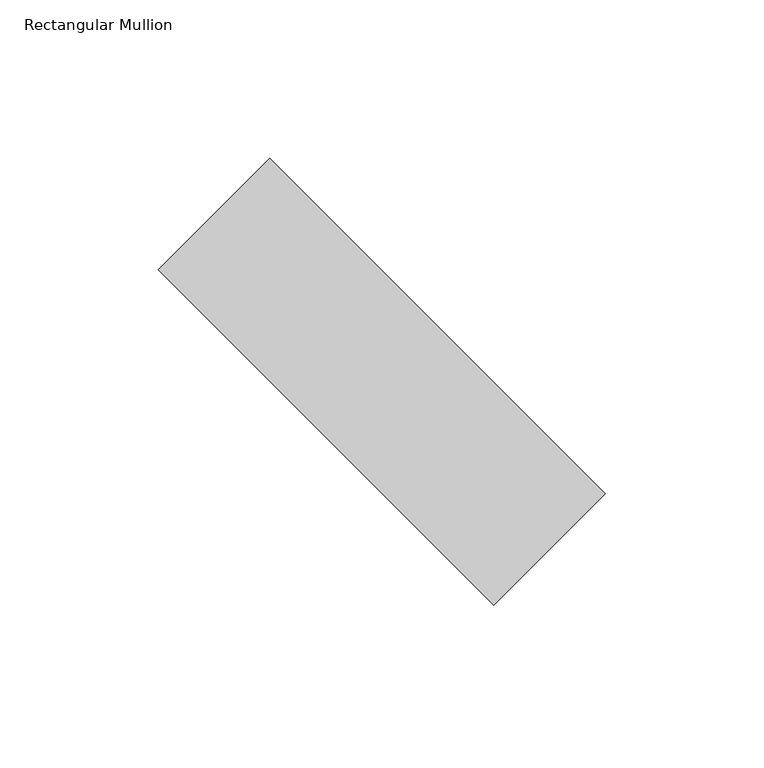
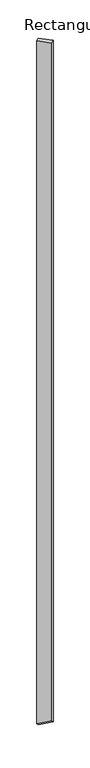
"""IFC4 building model written with IfcOpenShell, lengths in millimetres: member geometry, Rectangular Mullion : tilted mullions."""

from ifc_helpers import new_model, si_unit, origin, place, context, project, spatial, faceted_brep, source, transform, mapped, element, save


def rectangular_mullion_89872d6a(model_context):
    return source(origin(), model_context, "Body", "Brep", [
        faceted_brep([(-35.3553391, 70.7106781, 0.0), (-70.7106781, 35.3553391, 0.0), (35.3553391, -70.7106781, 0.0), (70.7106781, -35.3553391, 0.0), (-35.3553391, 70.7106781, -8054.9026078), (-70.7106781, 35.3553391, -8009.8417368), (35.3553391, -70.7106781, -7944.8366513), (70.7106781, -35.3553391, -7989.8975224)], [[[0, 1, 2, 3]], [[1, 0, 4, 5]], [[2, 1, 5, 6]], [[3, 2, 6, 7]], [[0, 3, 7, 4]], [[4, 7, 6, 5]]]),
    ])


if __name__ == "__main__":
    model = new_model("IFC4")
    model_context = context("Model", 3, world=origin())
    ifc_project = project(units=[si_unit("LENGTHUNIT", "METRE", prefix="MILLI")], contexts=[model_context])
    site = spatial("IfcSite", under=ifc_project)
    building = spatial("IfcBuilding", under=site)
    placement = place(None, origin())
    rectangular_mullion_shape = rectangular_mullion_89872d6a(model_context)
    element("IfcMember", 1, ObjectType="Rectangular Mullion : tilted mullions", at=placement, inside=building, context=model_context, shape_type="MappedRepresentation", body=[
        mapped(rectangular_mullion_shape, transform((0.0, 0.0, 0.0), x_axis=(1.0, 0.0, 0.0), y_axis=(0.0, 1.0, 0.0), z_axis=(0.0, 0.0, 1.0))),
    ])
    save(model, "model.ifc")

# Revit data of these elements
# Type "Rectangular Mullion : tilted mullions"
#   built-in parameter 1007304 = 0.492126 (stored number, unit not read)
#   built-in parameter 1007301 = 0.082021 (stored number, unit not read)
#   built-in parameter 1007300 = 0.082021 (stored number, unit not read)
# Element 1 (IfcMember, "Rectangular Mullion : tilted mullions")
#   Materials on its faces: "Aluminum"
# Materials
#   "Aluminum": class "Metal", colour RGB 244 244 244, transparency 0, Description = "Aluminum 6061", Cost = 0
